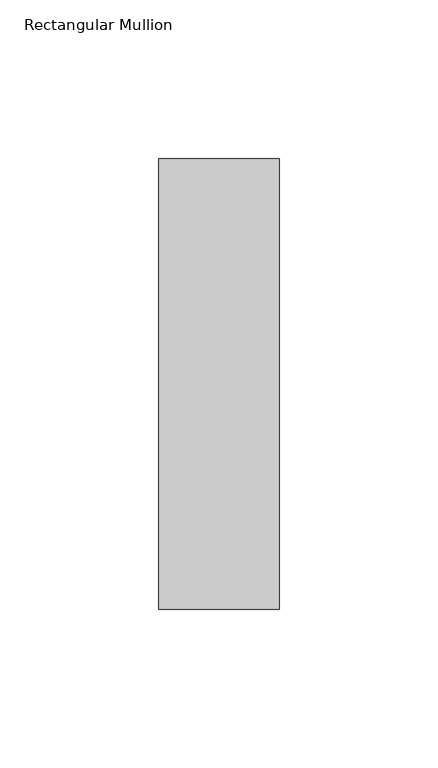
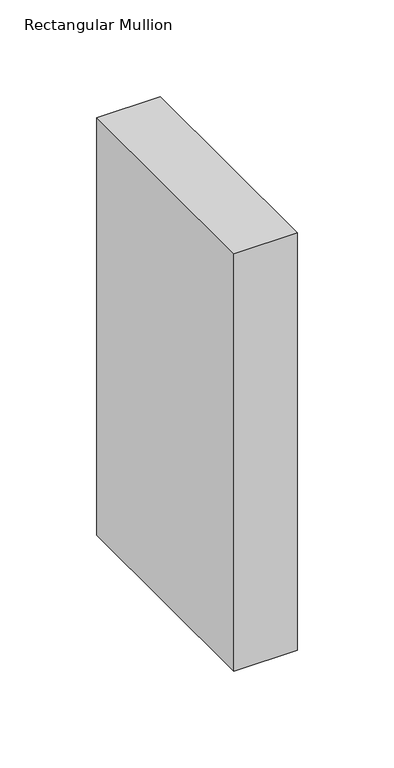
"""IFC4 building model written with IfcOpenShell, lengths in millimetres: member geometry, Rectangular Mullion : NLRS_21_CWM_hsb-regel 38x142_gen_rsf."""

from ifc_helpers import new_model, si_unit, frame, origin, place, context, project, spatial, polyline, outline, extrude, source, transform, mapped, element, save


def rectangular_mullion_c3680573(model_context):
    return source(origin(), model_context, "Body", "SweptSolid", [
        extrude(outline(polyline([(-38.0, -71.0), (-38.0, 71.0), (0.0, 71.0), (0.0, -71.0), (-38.0, -71.0)])), frame((0.0, 0.0, -264.0000003), z_axis=(0.0, 0.0, 1.0), x_axis=(1.0, 0.0, 0.0)), (0.0, 0.0, 1.0), 264.0000003),
    ])


if __name__ == "__main__":
    model = new_model("IFC4")
    model_context = context("Model", 3, world=origin())
    ifc_project = project(units=[si_unit("LENGTHUNIT", "METRE", prefix="MILLI")], contexts=[model_context])
    site = spatial("IfcSite", under=ifc_project)
    building = spatial("IfcBuilding", under=site)
    placement = place(None, origin())
    rectangular_mullion_shape = rectangular_mullion_c3680573(model_context)
    element("IfcMember", 1, ObjectType="Rectangular Mullion : NLRS_21_CWM_hsb-regel 38x142_gen_rsf", at=placement, inside=building, context=model_context, shape_type="MappedRepresentation", body=[
        mapped(rectangular_mullion_shape, transform((0.0, 0.0, 0.0), x_axis=(1.0, 0.0, 0.0), y_axis=(0.0, 1.0, 0.0), z_axis=(0.0, 0.0, 1.0))),
    ])
    save(model, "model.ifc")

# Revit data of these elements
# Type "Rectangular Mullion : NLRS_21_CWM_hsb-regel 38x142_gen_rsf"
#   Export Type to IFC As = "IfcWall"
#   Type IfcGUID = "07M7mRoiH1CR8m_RSKIwpF"
#   Assembly Code = "21.10"
#   built-in parameter 1007322 = 0.465879 (stored number, unit not read)
#   built-in parameter 1007321 = 0.062336 (stored number, unit not read)
#   built-in parameter 1007320 = 0.062336 (stored number, unit not read)
# Element 1 (IfcMember, "Rectangular Mullion : NLRS_21_CWM_hsb-regel 38x142_gen_rsf")
#   Materials on its faces: "NLRS_i2_hout naaldhout vuren_gen_rsf"
# Materials
#   "NLRS_i2_hout naaldhout vuren_gen_rsf": class "I - Hout", colour RGB 234 199 147, transparency 0, Keynote = "i2", Manufacturer = "Revit Standards Foundation", URL = "www.revitstandards.org", Description = "hout vuren", Cost = 0
